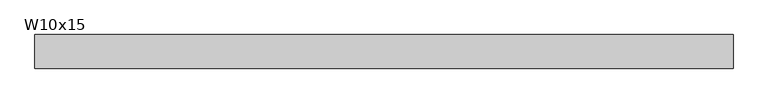
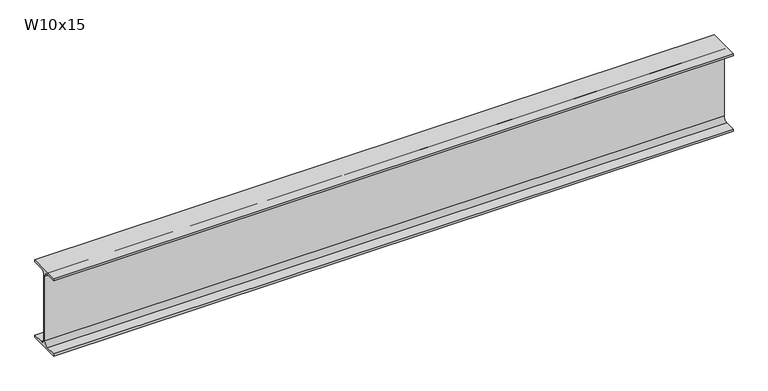
"""IFC4 building model written with IfcOpenShell, lengths in millimetres: beam geometry, RME W-Wide Flange : W10x15."""

from ifc_helpers import new_model, si_unit, point, frame, frame_2d, origin, place, context, project, spatial, polyline, circle_curve, trimmed, segment, composite_curve, outline, extrude, source, transform, mapped, element, save


def w10x15_c6b557fc(model_context):
    return source(origin(), model_context, "Body", "SweptSolid", [
        extrude(outline(composite_curve([segment(polyline([(50.8, -120.142), (50.8, -127.0), (-50.8, -127.0), (-50.8, -120.142), (-16.7005, -120.142)]), True, "CONTINUOUS"), segment(trimmed(circle_curve(frame_2d((-16.7005, -106.3625)), 13.7795), [point((-16.7005, -120.142))], [point((-2.921, -106.3625))], True, "CARTESIAN"), True, "CONTINUOUS"), segment(polyline([(-2.921, -106.3625), (-2.921, 106.3625)]), True, "CONTINUOUS"), segment(trimmed(circle_curve(frame_2d((-16.7005, 106.3625)), 13.7795), [point((-2.921, 106.3625))], [point((-16.7005, 120.142))], True, "CARTESIAN"), True, "CONTINUOUS"), segment(polyline([(-16.7005, 120.142), (-50.8, 120.142), (-50.8, 127.0), (50.8, 127.0), (50.8, 120.142), (16.7005, 120.142)]), True, "CONTINUOUS"), segment(trimmed(circle_curve(frame_2d((16.7005, 106.3625)), 13.7795), [point((16.7005, 120.142))], [point((2.921, 106.3625))], True, "CARTESIAN"), True, "CONTINUOUS"), segment(polyline([(2.921, 106.3625), (2.921, -106.3625)]), True, "CONTINUOUS"), segment(trimmed(circle_curve(frame_2d((16.7005, -106.3625)), 13.7795), [point((2.921, -106.3625))], [point((16.7005, -120.142))], True, "CARTESIAN"), True, "CONTINUOUS"), segment(polyline([(16.7005, -120.142), (50.8, -120.142)]), True, "CONTINUOUS")], self_intersect=False)), frame((-1054.1, 0.0, 0.0), z_axis=(1.0, 0.0, 0.0), x_axis=(0.0, 1.0, 0.0)), (0.0, 0.0, 1.0), 2108.2),
    ])


if __name__ == "__main__":
    model = new_model("IFC4")
    model_context = context("Model", 3, world=origin())
    ifc_project = project(units=[si_unit("LENGTHUNIT", "METRE", prefix="MILLI")], contexts=[model_context])
    site = spatial("IfcSite", under=ifc_project)
    building = spatial("IfcBuilding", under=site)
    placement = place(None, origin())
    w10x15_shape = w10x15_c6b557fc(model_context)
    element("IfcBeam", 1, ObjectType="RME W-Wide Flange : W10x15", at=placement, inside=building, context=model_context, shape_type="MappedRepresentation", body=[
        mapped(w10x15_shape, transform((0.0, 0.0, 0.0), x_axis=(1.0, 0.0, 0.0), y_axis=(0.0, 1.0, 0.0), z_axis=(0.0, 0.0, 1.0))),
    ])
    save(model, "model.ifc")

# Revit data of these elements
# Type "RME W-Wide Flange : W10x15"
#   WELD P [instance default] = ""
#   WELD LE [instance default] = ""
#   WELD D [instance default] = ""
#   TOP SECTION SIZE [instance default] = ""
#   TOP SECTION LENGTH [instance default] = ""
#   REMARKS [instance default] = ""
#   REINF TYPE [instance default] = ""
#   Nominal Size = "W24"
#   End Bearing Capacity [instance default] = ""
#   BOT SECTION SIZE [instance default] = ""
#   BOT SECTION LENGTH [instance default] = ""
#   Assembly Code = "B10"
#   W = 15
#   Start Extension Calculation [instance default] = 10' - 0"
#   Start Extension [instance default] = -0' - 0 1/2"
#   End Extension Calculation [instance default] = 10' - 0"
#   End Extension [instance default] = -0' - 0 1/2"
#   Length [instance default] = 5' - 0"
#   bf = 0' - 4"
#   d = 0' - 10"
#   k = 0' - 0 13/16"
#   k2 = 0' - 0.5425"
#   tf = 0' - 0.27"
#   tw = 0' - 0.23"
#   A = 0.030625 SF
#   Structural Material [instance default] = Metal - Steel - ASTM A992
# Element 1 (IfcBeam, "RME W-Wide Flange : W10x15")
#   Length = 6' - 11"
#   Materials on its faces: "Metal - Steel - ASTM A992"
# Materials
#   "Metal - Steel - ASTM A992": class "Metal", colour RGB 255 128 0, transparency 0
